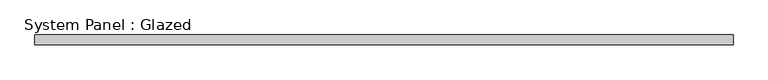
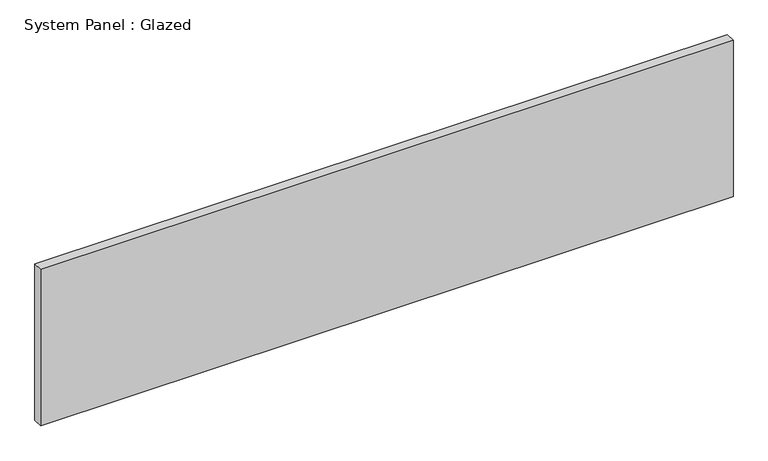
"""IFC4 building model written with IfcOpenShell, lengths in millimetres: plate geometry, System Panel : Glazed."""

from ifc_helpers import new_model, si_unit, origin, origin_with_axes, place, context, project, spatial, polyline, outline, extrude, source, transform, mapped, element, save


def system_panel_glazed_fa1c4aa4(model_context):
    return source(origin(), model_context, "Body", "SweptSolid", [
        extrude(outline(polyline([(890.0, -49.5), (-890.0, -49.5), (-890.0, -24.5), (890.0, -24.5), (890.0, -49.5)])), origin_with_axes(), (0.0, 0.0, 1.0), 425.0),
    ])


if __name__ == "__main__":
    model = new_model("IFC4")
    model_context = context("Model", 3, world=origin())
    ifc_project = project(units=[si_unit("LENGTHUNIT", "METRE", prefix="MILLI")], contexts=[model_context])
    site = spatial("IfcSite", under=ifc_project)
    building = spatial("IfcBuilding", under=site)
    placement = place(None, origin())
    system_panel_glazed_shape = system_panel_glazed_fa1c4aa4(model_context)
    element("IfcPlate", 1, ObjectType="System Panel : Glazed", at=placement, inside=building, context=model_context, shape_type="MappedRepresentation", body=[
        mapped(system_panel_glazed_shape, transform((0.0, 0.0, 0.0), x_axis=(1.0, 0.0, 0.0), y_axis=(0.0, 1.0, 0.0), z_axis=(0.0, 0.0, 1.0))),
    ])
    save(model, "model.ifc")

# Revit data of these elements
# Type "System Panel : Glazed"
#   Keynote = "H11"
#   Construction Type Id = "GSP4R"
#   Analytic Construction = "1/8 in Pilkington single glazing"
#   Visual Light Transmittance = 0.9
#   Solar Heat Gain Coefficient = 0.86
#   Heat Transfer Coefficient (U) = 6.7069 W/(m²·K)
# Element 1 (IfcPlate, "System Panel : Glazed")
#   Materials on its faces: "Glass"
# Materials
#   "Glass": class "Glass", colour RGB 0 128 192, transparency 0.9, Description = "Soda Lime Glass", Cost = 0
